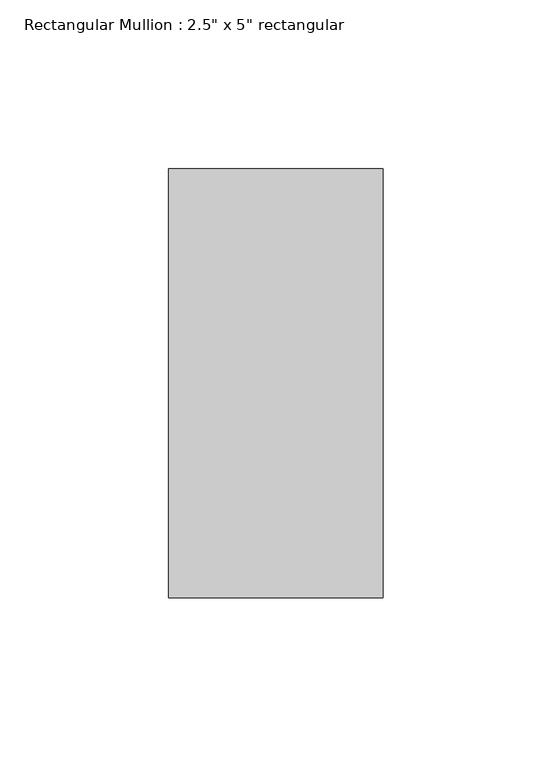
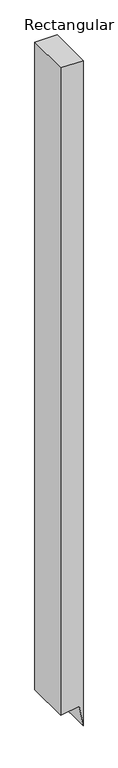
"""IFC4 building model written with IfcOpenShell, lengths in millimetres: member geometry."""

from ifc_helpers import new_model, si_unit, frame, origin, place, context, project, spatial, polyline, outline, extrude, source, transform, mapped, element, save


def member_19a11b55(model_context):
    return source(origin(), model_context, "Body", "SweptSolid", [
        extrude(outline(polyline([(0.0, 0.0), (0.0, -63.5), (-1944.3398442, -63.5), (-1935.0873785, -11.0266593), (-1997.6226708, 0.0), (0.0, 0.0)])), frame((0.0, -63.5, 0.0), z_axis=(0.0, 1.0, 0.0), x_axis=(0.0, 0.0, 1.0)), (0.0, 0.0, 1.0), 127.0),
    ])


if __name__ == "__main__":
    model = new_model("IFC4")
    model_context = context("Model", 3, world=origin())
    ifc_project = project(units=[si_unit("LENGTHUNIT", "METRE", prefix="MILLI")], contexts=[model_context])
    site = spatial("IfcSite", under=ifc_project)
    building = spatial("IfcBuilding", under=site)
    placement = place(None, origin())
    member_shape = member_19a11b55(model_context)
    element("IfcMember", 1, ObjectType="Rectangular Mullion : 2.5\" x 5\" rectangular", at=placement, inside=building, context=model_context, shape_type="MappedRepresentation", body=[
        mapped(member_shape, transform((0.0, 0.0, 0.0), x_axis=(1.0, 0.0, 0.0), y_axis=(0.0, 1.0, 0.0), z_axis=(0.0, 0.0, 1.0))),
    ])
    save(model, "model.ifc")

# Revit data of these elements
# Type "Rectangular Mullion : 2.5\" x 5\" rectangular"
#   built-in parameter 1007304 = 0.416667 (stored number, unit not read)
#   built-in parameter 1007301 = 0.104167 (stored number, unit not read)
#   built-in parameter 1007300 = 0.104167 (stored number, unit not read)
# Element 1 (IfcMember, "Rectangular Mullion : 2.5\" x 5\" rectangular")
#   Materials on its faces: "Black Mullions"
# Materials
#   "Black Mullions": class "Wood", colour RGB 0 0 0, transparency 0, Cost = 0
